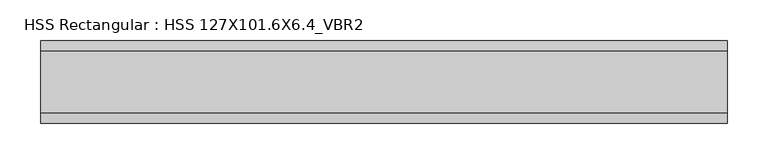
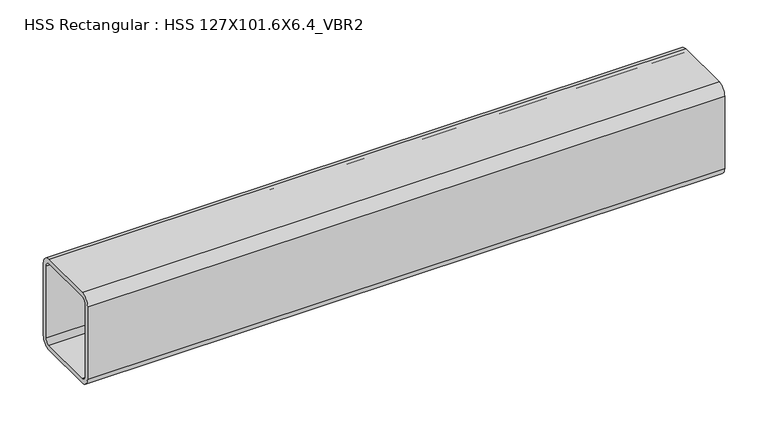
"""IFC4 building model written with IfcOpenShell, lengths in millimetres: member geometry, HSS Rectangular : HSS 127X101.6X6.4_VBR2."""

import ifcopenshell
import ifcopenshell.guid

model = None  # the IFC model being written
_history = None  # IfcOwnerHistory: only IFC2X3 demands one
_inside = {}  # id of a spatial element -> (the spatial element, [elements in it])
_under = {}  # id of a project, library or spatial element -> (it, [spatial elements below it])
_declared = {}  # id of a project -> (the project, [libraries it declares])
_typed = {}  # id of a type object -> (the type object, [elements of that type])
_made_of = {}  # id of a material, layer set ... -> (it, [elements and type objects made of it])


def new_model(schema):
    """Start an empty IFC model of exactly this schema.

    Asked for "IFC4X3", IfcOpenShell would pick the latest addendum, in which some entities
    have other attributes; the version numbers below select the first issue.
    IFC2X3 requires an IfcOwnerHistory on every rooted entity: one is made here for all.
    """
    global model, _history
    if schema == "IFC4X3":
        model = ifcopenshell.file(schema_version=(4, 3, 0, 0))
    else:
        model = ifcopenshell.file(schema=schema)
    _inside.clear()
    _under.clear()
    _declared.clear()
    _typed.clear()
    _made_of.clear()
    _history = None
    if model.schema == "IFC2X3":
        org = make("IfcOrganization", Name="unknown")
        user = make(
            "IfcPersonAndOrganization",
            ThePerson=make("IfcPerson", FamilyName="unknown"),
            TheOrganization=org,
        )
        app = make(
            "IfcApplication",
            ApplicationDeveloper=org,
            Version="unknown",
            ApplicationFullName="unknown",
            ApplicationIdentifier="unknown",
        )
        _history = make(
            "IfcOwnerHistory",
            OwningUser=user,
            OwningApplication=app,
            ChangeAction="ADDED",
            CreationDate=0,
        )
    return model


def make(cls, **values):
    """One entity of the class cls with the attributes given. An attribute that is None is left unset."""
    return model.create_entity(
        cls, **{name: value for name, value in values.items() if value is not None}
    )


def rooted(cls, **values):
    """An entity with a GlobalId (a new one), such as an element, a storey or a relation."""
    return make(cls, GlobalId=ifcopenshell.guid.new(), OwnerHistory=_history, **values)


def si_unit(unit_type, name, prefix=None):
    """IfcSIUnit, for example si_unit("LENGTHUNIT", "METRE", prefix="MILLI")."""
    return make("IfcSIUnit", UnitType=unit_type, Prefix=prefix, Name=name)


def assignment(units):
    """IfcUnitAssignment: the units of a project."""
    return None if units is None else make("IfcUnitAssignment", Units=units)


def point(xyz):
    """IfcCartesianPoint."""
    return None if xyz is None else make("IfcCartesianPoint", Coordinates=xyz)


def direction(xyz):
    """IfcDirection."""
    return None if xyz is None else make("IfcDirection", DirectionRatios=xyz)


def frame(location, z_axis=None, x_axis=None):
    """IfcAxis2Placement3D, a coordinate frame: its origin and axes. An axis left out is left unset."""
    return make(
        "IfcAxis2Placement3D",
        Location=point(location),
        Axis=direction(z_axis),
        RefDirection=direction(x_axis),
    )


def frame_2d(location, x_axis=None):
    """IfcAxis2Placement2D, a coordinate frame in the plane: its origin and x axis."""
    return make(
        "IfcAxis2Placement2D", Location=point(location), RefDirection=direction(x_axis)
    )


def origin():
    """The frame at (0, 0, 0) with its axes left unset."""
    return frame((0.0, 0.0, 0.0))


def place(relative_to, where):
    """IfcLocalPlacement: puts the frame where relative to a parent placement (None: the world)."""
    return make(
        "IfcLocalPlacement", PlacementRelTo=relative_to, RelativePlacement=where
    )


def context(
    kind, dimensions, precision=None, world=None, true_north=None, identifier=None
):
    """IfcGeometricRepresentationContext, for example the 3D "Model" context."""
    return make(
        "IfcGeometricRepresentationContext",
        ContextIdentifier=identifier,
        ContextType=kind,
        CoordinateSpaceDimension=dimensions,
        Precision=precision,
        WorldCoordinateSystem=world,
        TrueNorth=true_north,
    )


def project(units=None, contexts=None):
    """IfcProject with its units and contexts."""
    return rooted(
        "IfcProject",
        Name="project",
        RepresentationContexts=contexts,
        UnitsInContext=assignment(units),
    )


def spatial(cls, under=None, at=None, **own):
    """A site, building, storey or space (cls), placed at a placement, below another one or the project."""
    s = rooted(cls, ObjectPlacement=at, **own)
    if under is not None:
        _under.setdefault(under.id(), (under, []))[1].append(s)
    return s


def polyline(points):
    """IfcPolyline through the points."""
    return make("IfcPolyline", Points=[point(p) for p in points])


def circle_curve(where, radius):
    """IfcCircle in the frame where."""
    return make("IfcCircle", Position=where, Radius=radius)


def trimmed(basis, trim1, trim2, sense, master):
    """IfcTrimmedCurve: the piece of a basis curve between two trims."""
    return make(
        "IfcTrimmedCurve",
        BasisCurve=basis,
        Trim1=trim1,
        Trim2=trim2,
        SenseAgreement=sense,
        MasterRepresentation=master,
    )


def segment(curve, same_sense, transition):
    """IfcCompositeCurveSegment."""
    return make(
        "IfcCompositeCurveSegment",
        Transition=transition,
        SameSense=same_sense,
        ParentCurve=curve,
    )


def composite_curve(segments, self_intersect=None):
    """IfcCompositeCurve: segments joined end to end."""
    return make("IfcCompositeCurve", Segments=segments, SelfIntersect=self_intersect)


def outline(outer, holes=None, kind="AREA"):
    """IfcArbitraryClosedProfileDef: a profile drawn as a closed curve; with holes, ...WithVoids."""
    if holes is None:
        return make("IfcArbitraryClosedProfileDef", ProfileType=kind, OuterCurve=outer)
    return make(
        "IfcArbitraryProfileDefWithVoids",
        ProfileType=kind,
        OuterCurve=outer,
        InnerCurves=holes,
    )


def extrude(swept, where, along, depth):
    """IfcExtrudedAreaSolid: the profile swept, set in the frame where, extruded along a direction by depth."""
    return make(
        "IfcExtrudedAreaSolid",
        SweptArea=swept,
        Position=where,
        ExtrudedDirection=direction(along),
        Depth=depth,
    )


def shape(context_of_items, identifier, shape_type, items):
    """IfcShapeRepresentation: the items that make up one representation, for example the "Body"."""
    return make(
        "IfcShapeRepresentation",
        ContextOfItems=context_of_items,
        RepresentationIdentifier=identifier,
        RepresentationType=shape_type,
        Items=items,
    )


def source(mapping_origin, context_of_items, identifier, shape_type, items):
    """IfcRepresentationMap: a shape defined once, which mapped items show again and again."""
    return make(
        "IfcRepresentationMap",
        MappingOrigin=mapping_origin,
        MappedRepresentation=shape(context_of_items, identifier, shape_type, items),
    )


def transform(
    local_origin,
    x_axis=None,
    y_axis=None,
    z_axis=None,
    scale=None,
    scale2=None,
    scale3=None,
    uniform=True,
):
    """IfcCartesianTransformationOperator3D, or its non-uniform kind. x_axis, y_axis, z_axis: its Axis1, 2, 3."""
    if uniform:
        return make(
            "IfcCartesianTransformationOperator3D",
            Axis1=direction(x_axis),
            Axis2=direction(y_axis),
            LocalOrigin=point(local_origin),
            Scale=scale,
            Axis3=direction(z_axis),
        )
    return make(
        "IfcCartesianTransformationOperator3DnonUniform",
        Axis1=direction(x_axis),
        Axis2=direction(y_axis),
        LocalOrigin=point(local_origin),
        Scale=scale,
        Axis3=direction(z_axis),
        Scale2=scale2,
        Scale3=scale3,
    )


def mapped(mapping_source, mapping_target):
    """IfcMappedItem: shows the shape of a source again, moved by a transform."""
    return make(
        "IfcMappedItem", MappingSource=mapping_source, MappingTarget=mapping_target
    )


def made_of(thing, what):
    """Note that an element or type object is made of a material, layer set ...; save() writes the relation."""
    if what is not None:
        _made_of.setdefault(what.id(), (what, []))[1].append(thing)
    return thing


def element(
    cls,
    number,
    at=None,
    inside=None,
    cuts=None,
    type_object=None,
    material=None,
    context=None,
    identifier="Body",
    shape_type=None,
    held_by="IfcProductDefinitionShape",
    body=None,
    shapes=None,
    **own,
):
    """One element of the class cls, such as IfcWall. Its Tag is "e" and its number.

    at: its placement. inside: the storey or other place that contains it. cuts: it is an
    opening in that element (IfcRelVoidsElement). A single representation is given by context,
    identifier, shape_type and body (its items); several are given by shapes. held_by: the class
    of the entity that holds the representations. save() writes the other relations.
    """
    e = rooted(cls, Tag="e%d" % number, ObjectPlacement=at, **own)
    if body is not None:
        shapes = [shape(context, identifier, shape_type, body)]
    if shapes is not None:
        e.Representation = make(held_by, Representations=shapes)
    if inside is not None:
        _inside.setdefault(inside.id(), (inside, []))[1].append(e)
    if cuts is not None:
        rooted(
            "IfcRelVoidsElement", RelatingBuildingElement=cuts, RelatedOpeningElement=e
        )
    if type_object is not None:
        _typed.setdefault(type_object.id(), (type_object, []))[1].append(e)
    return made_of(e, material)


def aggregate(whole, parts):
    """IfcRelAggregates: a whole, such as a stair, and the parts it consists of."""
    return rooted("IfcRelAggregates", RelatingObject=whole, RelatedObjects=parts)


def save(model, path):
    """Write the relations noted so far, then the file.

    IfcRelAggregates (storeys below a building ...), IfcRelContainedInSpatialStructure (elements
    in a storey), IfcRelDefinesByType, IfcRelAssociatesMaterial and IfcRelDeclares: one each for
    every whole, place, type object, material and project.
    """
    for whole, parts in _under.values():
        aggregate(whole, parts)
    for where, things in _inside.values():
        rooted(
            "IfcRelContainedInSpatialStructure",
            RelatedElements=things,
            RelatingStructure=where,
        )
    for kind, things in _typed.values():
        rooted("IfcRelDefinesByType", RelatedObjects=things, RelatingType=kind)
    for what, things in _made_of.values():
        rooted("IfcRelAssociatesMaterial", RelatedObjects=things, RelatingMaterial=what)
    for by, libraries in _declared.values():
        rooted("IfcRelDeclares", RelatingContext=by, RelatedDefinitions=libraries)
    model.write(path)


def hss_rectangular_hss_127x101_6x6_4_vbr2_ca43d79c(model_context):
    return source(origin(), model_context, "Body", "SweptSolid", [
        extrude(outline(composite_curve([segment(polyline([(50.8, 50.8), (50.8, -50.8)]), True, "CONTINUOUS"), segment(trimmed(circle_curve(frame_2d((38.1, -50.8)), 12.7), [point((50.8, -50.8))], [point((38.1, -63.5))], False, "CARTESIAN"), True, "CONTINUOUS"), segment(polyline([(38.1, -63.5), (-38.1, -63.5)]), True, "CONTINUOUS"), segment(trimmed(circle_curve(frame_2d((-38.1, -50.8)), 12.7), [point((-38.1, -63.5))], [point((-50.8, -50.8))], False, "CARTESIAN"), True, "CONTINUOUS"), segment(polyline([(-50.8, -50.8), (-50.8, 50.8)]), True, "CONTINUOUS"), segment(trimmed(circle_curve(frame_2d((-38.1, 50.8)), 12.7), [point((-50.8, 50.8))], [point((-38.1, 63.5))], False, "CARTESIAN"), True, "CONTINUOUS"), segment(polyline([(-38.1, 63.5), (38.1, 63.5)]), True, "CONTINUOUS"), segment(trimmed(circle_curve(frame_2d((38.1, 50.8)), 12.7), [point((38.1, 63.5))], [point((50.8, 50.8))], False, "CARTESIAN"), True, "CONTINUOUS")], self_intersect=False), holes=[composite_curve([segment(trimmed(circle_curve(frame_2d((-38.1, 50.8)), 6.35), [point((-38.1, 57.15))], [point((-44.45, 50.8))], True, "CARTESIAN"), True, "CONTINUOUS"), segment(polyline([(-44.45, 50.8), (-44.45, -50.8)]), True, "CONTINUOUS"), segment(trimmed(circle_curve(frame_2d((-38.1, -50.8)), 6.35), [point((-44.45, -50.8))], [point((-38.1, -57.15))], True, "CARTESIAN"), True, "CONTINUOUS"), segment(polyline([(-38.1, -57.15), (38.1, -57.15)]), True, "CONTINUOUS"), segment(trimmed(circle_curve(frame_2d((38.1, -50.8)), 6.35), [point((38.1, -57.15))], [point((44.45, -50.8))], True, "CARTESIAN"), True, "CONTINUOUS"), segment(polyline([(44.45, -50.8), (44.45, 50.8)]), True, "CONTINUOUS"), segment(trimmed(circle_curve(frame_2d((38.1, 50.8)), 6.35), [point((44.45, 50.8))], [point((38.1, 57.15))], True, "CARTESIAN"), True, "CONTINUOUS"), segment(polyline([(38.1, 57.15), (-38.1, 57.15)]), True, "CONTINUOUS")], self_intersect=False)]), frame((-368.3061368, 0.0, 0.0), z_axis=(1.0, 0.0, 0.0), x_axis=(0.0, 1.0, 0.0)), (0.0, 0.0, 1.0), 846.4945254),
    ])


if __name__ == "__main__":
    model = new_model("IFC4")
    model_context = context("Model", 3, world=origin())
    ifc_project = project(units=[si_unit("LENGTHUNIT", "METRE", prefix="MILLI")], contexts=[model_context])
    site = spatial("IfcSite", under=ifc_project)
    building = spatial("IfcBuilding", under=site)
    placement = place(None, origin())
    hss_rectangular_hss_127x101_6x6_4_vbr2_shape = hss_rectangular_hss_127x101_6x6_4_vbr2_ca43d79c(model_context)
    element("IfcMember", 1, ObjectType="HSS Rectangular : HSS 127X101.6X6.4_VBR2", at=placement, inside=building, context=model_context, shape_type="MappedRepresentation", body=[
        mapped(hss_rectangular_hss_127x101_6x6_4_vbr2_shape, transform((0.0, 0.0, 0.0), x_axis=(1.0, 0.0, 0.0), y_axis=(0.0, 1.0, 0.0), z_axis=(0.0, 0.0, 1.0))),
    ])
    save(model, "model.ifc")

# Revit data of these elements
# Type "HSS Rectangular : HSS 127X101.6X6.4_VBR2"
#   Section Name Key = "HSS5X4X1/4"
#   Assembly Code = "B10"
#   Width = 10.16 cm
#   Wall Nominal Thickness = 0.635 cm
#   Wall Design Thickness = 0.5918 cm
#   Torsional Moment of Inertia = 749.217 cm⁴
#   Torsional Modulus = 136.34 cm³
#   Section Area = 24.7741 cm²
#   Plastic Modulus weak axis = 91.2759 cm³
#   Plastic Modulus strong axis = 106.352 cm³
#   Perimeter = 0.435254 m²/m
#   Outer Fillet = 1.27 cm
#   Nominal Weight = 20.7004 kgf/m
#   Moment of Inertia weak axis = 393.755 cm⁴
#   Moment of Inertia strong axis = 557.75 cm⁴
#   Inner Fillet = 0.635 cm
#   Height = 12.7 cm
#   Elastic Modulus weak axis = 77.5108 cm³
#   Elastic Modulus strong axis = 87.6708 cm³
#   Centroid Vertical = 6.35 cm
#   Centroid Horizontal = 5.08 cm
#   Length [instance default] = 1524 mm
#   Structural Material [instance default] = Steel ASTM A500, Grade C, Rectangular and Square
#   Principal Axes Angle = 0
# Element 1 (IfcMember, "HSS Rectangular : HSS 127X101.6X6.4_VBR2")
#   Materials on its faces: "Steel ASTM A500, Grade C, Rectangular and Square"
# Materials
#   "Steel ASTM A500, Grade C, Rectangular and Square": class "Metal", colour RGB 120 120 120, transparency 0, Description = "Carbon steel", Cost = 0
